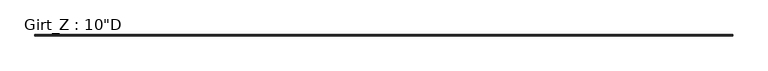
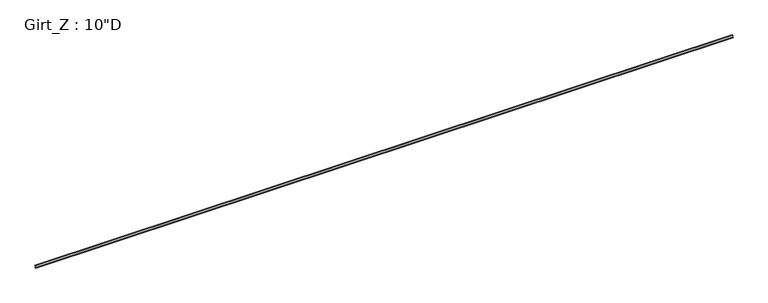
"""IFC4 building model written with IfcOpenShell, lengths in millimetres: beam geometry."""

import ifcopenshell
import ifcopenshell.guid

model = None  # the IFC model being written
_history = None  # IfcOwnerHistory: only IFC2X3 demands one
_inside = {}  # id of a spatial element -> (the spatial element, [elements in it])
_under = {}  # id of a project, library or spatial element -> (it, [spatial elements below it])
_declared = {}  # id of a project -> (the project, [libraries it declares])
_typed = {}  # id of a type object -> (the type object, [elements of that type])
_made_of = {}  # id of a material, layer set ... -> (it, [elements and type objects made of it])


def new_model(schema):
    """Start an empty IFC model of exactly this schema.

    Asked for "IFC4X3", IfcOpenShell would pick the latest addendum, in which some entities
    have other attributes; the version numbers below select the first issue.
    IFC2X3 requires an IfcOwnerHistory on every rooted entity: one is made here for all.
    """
    global model, _history
    if schema == "IFC4X3":
        model = ifcopenshell.file(schema_version=(4, 3, 0, 0))
    else:
        model = ifcopenshell.file(schema=schema)
    _inside.clear()
    _under.clear()
    _declared.clear()
    _typed.clear()
    _made_of.clear()
    _history = None
    if model.schema == "IFC2X3":
        org = make("IfcOrganization", Name="unknown")
        user = make(
            "IfcPersonAndOrganization",
            ThePerson=make("IfcPerson", FamilyName="unknown"),
            TheOrganization=org,
        )
        app = make(
            "IfcApplication",
            ApplicationDeveloper=org,
            Version="unknown",
            ApplicationFullName="unknown",
            ApplicationIdentifier="unknown",
        )
        _history = make(
            "IfcOwnerHistory",
            OwningUser=user,
            OwningApplication=app,
            ChangeAction="ADDED",
            CreationDate=0,
        )
    return model


def make(cls, **values):
    """One entity of the class cls with the attributes given. An attribute that is None is left unset."""
    return model.create_entity(
        cls, **{name: value for name, value in values.items() if value is not None}
    )


def rooted(cls, **values):
    """An entity with a GlobalId (a new one), such as an element, a storey or a relation."""
    return make(cls, GlobalId=ifcopenshell.guid.new(), OwnerHistory=_history, **values)


def si_unit(unit_type, name, prefix=None):
    """IfcSIUnit, for example si_unit("LENGTHUNIT", "METRE", prefix="MILLI")."""
    return make("IfcSIUnit", UnitType=unit_type, Prefix=prefix, Name=name)


def assignment(units):
    """IfcUnitAssignment: the units of a project."""
    return None if units is None else make("IfcUnitAssignment", Units=units)


def point(xyz):
    """IfcCartesianPoint."""
    return None if xyz is None else make("IfcCartesianPoint", Coordinates=xyz)


def direction(xyz):
    """IfcDirection."""
    return None if xyz is None else make("IfcDirection", DirectionRatios=xyz)


def frame(location, z_axis=None, x_axis=None):
    """IfcAxis2Placement3D, a coordinate frame: its origin and axes. An axis left out is left unset."""
    return make(
        "IfcAxis2Placement3D",
        Location=point(location),
        Axis=direction(z_axis),
        RefDirection=direction(x_axis),
    )


def frame_2d(location, x_axis=None):
    """IfcAxis2Placement2D, a coordinate frame in the plane: its origin and x axis."""
    return make(
        "IfcAxis2Placement2D", Location=point(location), RefDirection=direction(x_axis)
    )


def origin():
    """The frame at (0, 0, 0) with its axes left unset."""
    return frame((0.0, 0.0, 0.0))


def place(relative_to, where):
    """IfcLocalPlacement: puts the frame where relative to a parent placement (None: the world)."""
    return make(
        "IfcLocalPlacement", PlacementRelTo=relative_to, RelativePlacement=where
    )


def context(
    kind, dimensions, precision=None, world=None, true_north=None, identifier=None
):
    """IfcGeometricRepresentationContext, for example the 3D "Model" context."""
    return make(
        "IfcGeometricRepresentationContext",
        ContextIdentifier=identifier,
        ContextType=kind,
        CoordinateSpaceDimension=dimensions,
        Precision=precision,
        WorldCoordinateSystem=world,
        TrueNorth=true_north,
    )


def project(units=None, contexts=None):
    """IfcProject with its units and contexts."""
    return rooted(
        "IfcProject",
        Name="project",
        RepresentationContexts=contexts,
        UnitsInContext=assignment(units),
    )


def spatial(cls, under=None, at=None, **own):
    """A site, building, storey or space (cls), placed at a placement, below another one or the project."""
    s = rooted(cls, ObjectPlacement=at, **own)
    if under is not None:
        _under.setdefault(under.id(), (under, []))[1].append(s)
    return s


def polyline(points):
    """IfcPolyline through the points."""
    return make("IfcPolyline", Points=[point(p) for p in points])


def circle_curve(where, radius):
    """IfcCircle in the frame where."""
    return make("IfcCircle", Position=where, Radius=radius)


def trimmed(basis, trim1, trim2, sense, master):
    """IfcTrimmedCurve: the piece of a basis curve between two trims."""
    return make(
        "IfcTrimmedCurve",
        BasisCurve=basis,
        Trim1=trim1,
        Trim2=trim2,
        SenseAgreement=sense,
        MasterRepresentation=master,
    )


def segment(curve, same_sense, transition):
    """IfcCompositeCurveSegment."""
    return make(
        "IfcCompositeCurveSegment",
        Transition=transition,
        SameSense=same_sense,
        ParentCurve=curve,
    )


def composite_curve(segments, self_intersect=None):
    """IfcCompositeCurve: segments joined end to end."""
    return make("IfcCompositeCurve", Segments=segments, SelfIntersect=self_intersect)


def outline(outer, holes=None, kind="AREA"):
    """IfcArbitraryClosedProfileDef: a profile drawn as a closed curve; with holes, ...WithVoids."""
    if holes is None:
        return make("IfcArbitraryClosedProfileDef", ProfileType=kind, OuterCurve=outer)
    return make(
        "IfcArbitraryProfileDefWithVoids",
        ProfileType=kind,
        OuterCurve=outer,
        InnerCurves=holes,
    )


def extrude(swept, where, along, depth):
    """IfcExtrudedAreaSolid: the profile swept, set in the frame where, extruded along a direction by depth."""
    return make(
        "IfcExtrudedAreaSolid",
        SweptArea=swept,
        Position=where,
        ExtrudedDirection=direction(along),
        Depth=depth,
    )


def shape(context_of_items, identifier, shape_type, items):
    """IfcShapeRepresentation: the items that make up one representation, for example the "Body"."""
    return make(
        "IfcShapeRepresentation",
        ContextOfItems=context_of_items,
        RepresentationIdentifier=identifier,
        RepresentationType=shape_type,
        Items=items,
    )


def source(mapping_origin, context_of_items, identifier, shape_type, items):
    """IfcRepresentationMap: a shape defined once, which mapped items show again and again."""
    return make(
        "IfcRepresentationMap",
        MappingOrigin=mapping_origin,
        MappedRepresentation=shape(context_of_items, identifier, shape_type, items),
    )


def transform(
    local_origin,
    x_axis=None,
    y_axis=None,
    z_axis=None,
    scale=None,
    scale2=None,
    scale3=None,
    uniform=True,
):
    """IfcCartesianTransformationOperator3D, or its non-uniform kind. x_axis, y_axis, z_axis: its Axis1, 2, 3."""
    if uniform:
        return make(
            "IfcCartesianTransformationOperator3D",
            Axis1=direction(x_axis),
            Axis2=direction(y_axis),
            LocalOrigin=point(local_origin),
            Scale=scale,
            Axis3=direction(z_axis),
        )
    return make(
        "IfcCartesianTransformationOperator3DnonUniform",
        Axis1=direction(x_axis),
        Axis2=direction(y_axis),
        LocalOrigin=point(local_origin),
        Scale=scale,
        Axis3=direction(z_axis),
        Scale2=scale2,
        Scale3=scale3,
    )


def mapped(mapping_source, mapping_target):
    """IfcMappedItem: shows the shape of a source again, moved by a transform."""
    return make(
        "IfcMappedItem", MappingSource=mapping_source, MappingTarget=mapping_target
    )


def made_of(thing, what):
    """Note that an element or type object is made of a material, layer set ...; save() writes the relation."""
    if what is not None:
        _made_of.setdefault(what.id(), (what, []))[1].append(thing)
    return thing


def element(
    cls,
    number,
    at=None,
    inside=None,
    cuts=None,
    type_object=None,
    material=None,
    context=None,
    identifier="Body",
    shape_type=None,
    held_by="IfcProductDefinitionShape",
    body=None,
    shapes=None,
    **own,
):
    """One element of the class cls, such as IfcWall. Its Tag is "e" and its number.

    at: its placement. inside: the storey or other place that contains it. cuts: it is an
    opening in that element (IfcRelVoidsElement). A single representation is given by context,
    identifier, shape_type and body (its items); several are given by shapes. held_by: the class
    of the entity that holds the representations. save() writes the other relations.
    """
    e = rooted(cls, Tag="e%d" % number, ObjectPlacement=at, **own)
    if body is not None:
        shapes = [shape(context, identifier, shape_type, body)]
    if shapes is not None:
        e.Representation = make(held_by, Representations=shapes)
    if inside is not None:
        _inside.setdefault(inside.id(), (inside, []))[1].append(e)
    if cuts is not None:
        rooted(
            "IfcRelVoidsElement", RelatingBuildingElement=cuts, RelatedOpeningElement=e
        )
    if type_object is not None:
        _typed.setdefault(type_object.id(), (type_object, []))[1].append(e)
    return made_of(e, material)


def aggregate(whole, parts):
    """IfcRelAggregates: a whole, such as a stair, and the parts it consists of."""
    return rooted("IfcRelAggregates", RelatingObject=whole, RelatedObjects=parts)


def save(model, path):
    """Write the relations noted so far, then the file.

    IfcRelAggregates (storeys below a building ...), IfcRelContainedInSpatialStructure (elements
    in a storey), IfcRelDefinesByType, IfcRelAssociatesMaterial and IfcRelDeclares: one each for
    every whole, place, type object, material and project.
    """
    for whole, parts in _under.values():
        aggregate(whole, parts)
    for where, things in _inside.values():
        rooted(
            "IfcRelContainedInSpatialStructure",
            RelatedElements=things,
            RelatingStructure=where,
        )
    for kind, things in _typed.values():
        rooted("IfcRelDefinesByType", RelatedObjects=things, RelatingType=kind)
    for what, things in _made_of.values():
        rooted("IfcRelAssociatesMaterial", RelatedObjects=things, RelatingMaterial=what)
    for by, libraries in _declared.values():
        rooted("IfcRelDeclares", RelatingContext=by, RelatedDefinitions=libraries)
    model.write(path)


def beam_bf61a610(model_context):
    return source(origin(), model_context, "Body", "SweptSolid", [
        extrude(outline(composite_curve([segment(polyline([(77.9859375, 127.0), (90.2310415, 112.4068534), (88.1028742, 110.621109), (76.6904765, 124.221875), (3.3005807, 124.221875)]), True, "CONTINUOUS"), segment(trimmed(circle_curve(frame_2d((3.3741066, 122.2381931)), 1.9850441), [point((3.3005807, 124.221875))], [point((1.3890625, 122.2381931))], True, "CARTESIAN"), True, "CONTINUOUS"), segment(polyline([(1.3890625, 122.2381931), (1.3890625, -127.0), (-84.3359375, -127.0), (-96.5810415, -112.4068534), (-94.4528742, -110.621109), (-83.0404765, -124.221875), (-3.2694106, -124.221875)]), True, "CONTINUOUS"), segment(trimmed(circle_curve(frame_2d((-3.3748024, -122.2389339)), 1.9857399), [point((-3.2694106, -124.221875))], [point((-1.3890625, -122.2389339))], True, "CARTESIAN"), True, "CONTINUOUS"), segment(polyline([(-1.3890625, -122.2389339), (-1.3890625, 122.2375)]), True, "CONTINUOUS"), segment(trimmed(circle_curve(frame_2d((3.3734375, 122.2375)), 4.7625), [point((-1.3890625, 122.2375))], [point((3.3734375, 127.0))], False, "CARTESIAN"), True, "CONTINUOUS"), segment(polyline([(3.3734375, 127.0), (77.9859375, 127.0)]), True, "CONTINUOUS")], self_intersect=False)), frame((-44283.1884767, 0.0, 0.0), z_axis=(1.0, 0.0, 0.0), x_axis=(0.0, 1.0, 0.0)), (0.0, 0.0, 1.0), 88566.3769533),
    ])


if __name__ == "__main__":
    model = new_model("IFC4")
    model_context = context("Model", 3, world=origin())
    ifc_project = project(units=[si_unit("LENGTHUNIT", "METRE", prefix="MILLI")], contexts=[model_context])
    site = spatial("IfcSite", under=ifc_project)
    building = spatial("IfcBuilding", under=site)
    placement = place(None, origin())
    beam_shape = beam_bf61a610(model_context)
    element("IfcBeam", 1, ObjectType="Girt_Z : 10\"D", at=placement, inside=building, context=model_context, shape_type="MappedRepresentation", body=[
        mapped(beam_shape, transform((0.0, 0.0, 0.0), x_axis=(1.0, 0.0, 0.0), y_axis=(0.0, 1.0, 0.0), z_axis=(0.0, 0.0, 1.0))),
    ])
    save(model, "model.ifc")

# Revit data of these elements
# Type "Girt_Z : 10\"D"
#   half leg = 0' - 1 11/16"
#   Web_Thickness = 0' - 0 7/64"
#   Length [instance default] = 10' - 0"
#   Leg_2 = 0' - 3 3/8"
#   Leg_1 = 0' - 3 1/8"
#   Height = 0' - 10"
#   Structural Material [instance default] = none
# Element 1 (IfcBeam, "Girt_Z : 10\"D")
#   Structural Material = STRUCTURAL STEEL - SEE STRUCT. DWGS
#   Materials on its faces: "STRUCTURAL STEEL - SEE STRUCT. DWGS"
# Materials
#   "STRUCTURAL STEEL - SEE STRUCT. DWGS": class "Metal", colour RGB 137 146 153, transparency 0, Description = "Steel, mill finish", Cost = 0
